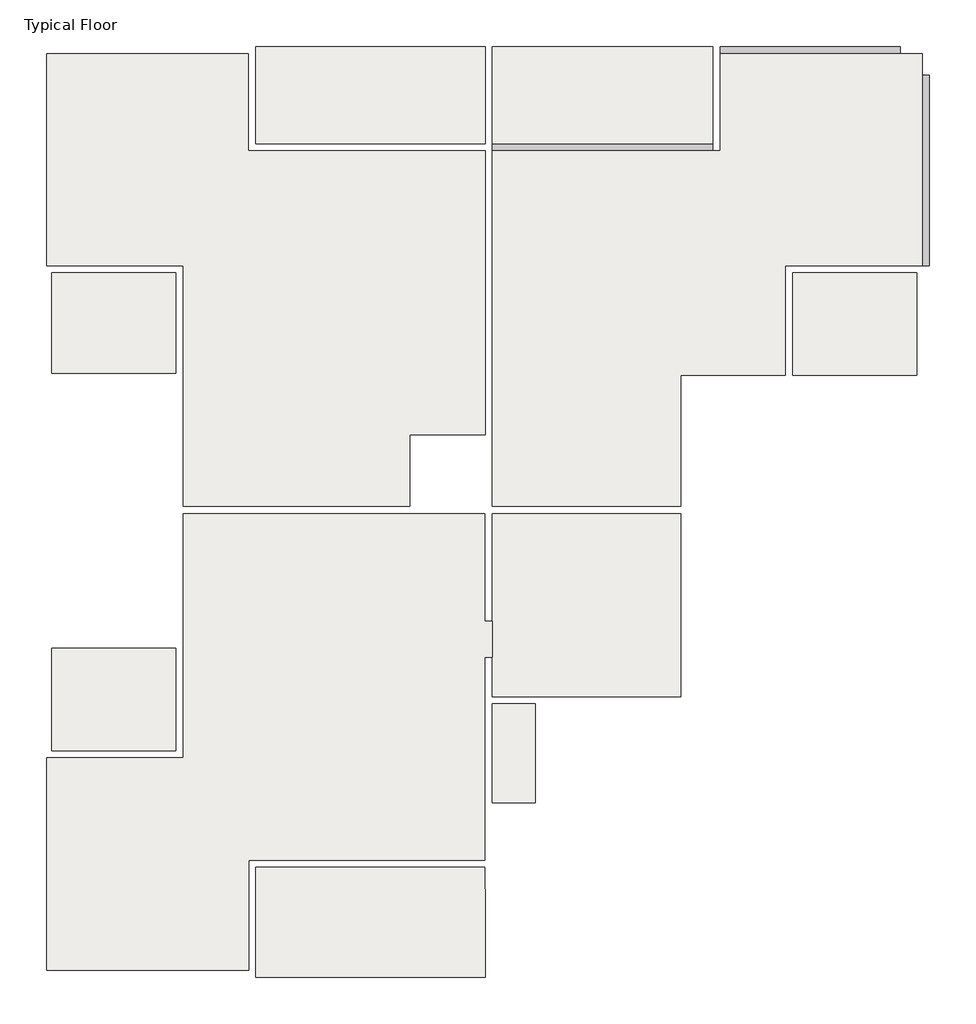
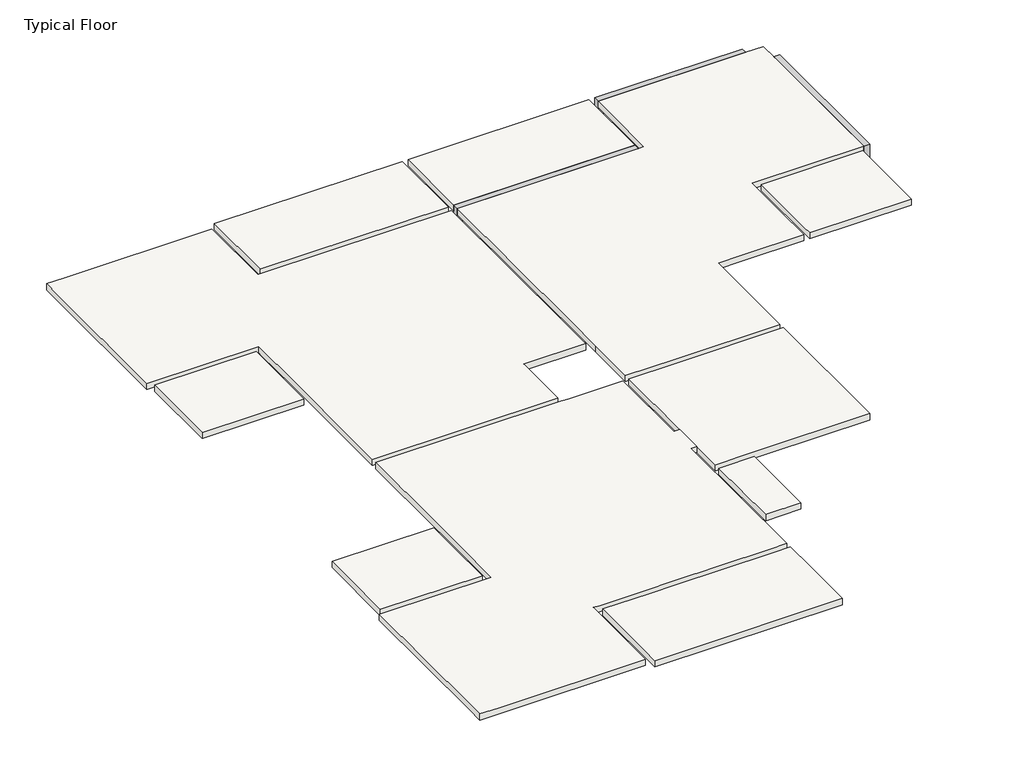
# One storey: 11 slabs, 3 beams.
"""IFC4 building model written with IfcOpenShell, lengths in millimetres."""

from ifc_helpers import new_model, si_unit, frame, origin, place, context, project, spatial, polyline, outline, extrude, faceted_brep, element, save

model = new_model("IFC4")

# Units and contexts
model_context = context("Model", 3, world=origin())
ifc_project = project(units=[si_unit("LENGTHUNIT", "METRE", prefix="MILLI")], contexts=[model_context])

# Site, building, storey
site = spatial("IfcSite", under=ifc_project)
building = spatial("IfcBuilding", under=site)
storey = spatial("IfcBuildingStorey", under=building, Name="Typical Floor", Elevation=3200.0)

# Beams
placement = place(None, origin())
element("IfcBeam", 1, ObjectType="Concrete Rectengular Beam : 20/50", at=placement, inside=storey, context=model_context, shape_type="Brep", body=[
    faceted_brep([(23241.1179501, 12375.8954895, 3200.0), (23241.1179501, 12575.8954895, 3200.0), (18221.404101, 12575.8954895, 3200.0), (18221.404101, 12375.8954895, 3200.0), (23241.1179501, 12375.8954895, 2700.0), (18221.404101, 12375.8954895, 2980.0), (18221.404101, 12375.8954895, 2700.0), (23241.1179501, 12575.8954895, 2700.0), (18221.404101, 12575.8954895, 2700.0)], [[[0, 1, 2, 3]], [[4, 0, 3, 5, 6]], [[7, 4, 6, 8]], [[1, 7, 8, 2]], [[1, 0, 4, 7]], [[3, 2, 8, 6, 5]]]),
])
element("IfcBeam", 2, ObjectType="Concrete Rectengular Beam : 20/50", at=placement, inside=storey, context=model_context, shape_type="Brep", body=[
    faceted_brep([(24041.1179501, 11775.8954895, 3200.0), (23841.1179501, 11775.8954895, 3200.0), (23841.1179501, 6476.2289939, 3200.0), (24041.1179501, 6476.2289939, 3200.0), (24041.1179501, 11775.8954895, 2700.0), (24041.1179501, 6476.2289939, 2700.0), (23841.1179501, 11775.8954895, 2700.0), (23841.1179501, 6476.2289939, 2700.0), (23841.1179501, 6476.2289939, 2980.0)], [[[0, 1, 2, 3]], [[4, 0, 3, 5]], [[6, 4, 5, 7]], [[1, 6, 7, 8, 2]], [[1, 0, 4, 6]], [[3, 2, 8, 7, 5]]]),
])
element("IfcBeam", 3, ObjectType="Concrete Rectengular Beam : 20/50", at=placement, inside=storey, context=model_context, shape_type="Brep", body=[
    faceted_brep([(11879.1824488, 9876.3316106, 3200.0), (11879.1824488, 9676.3316106, 3200.0), (18021.404101, 9676.3316106, 3200.0), (18021.404101, 9876.3316106, 3200.0), (11879.1824488, 9676.3316106, 2980.0), (11879.1824488, 9676.3316106, 2700.0), (18021.404101, 9676.3316106, 2700.0), (11879.1824488, 9876.3316106, 2700.0), (18021.404101, 9876.3316106, 2700.0), (11879.1824488, 9876.3316106, 2980.0), (18021.404101, 9876.3316106, 2980.0)], [[[0, 1, 2, 3]], [[1, 4, 5, 6, 2]], [[5, 7, 8, 6]], [[7, 9, 0, 3, 10, 8]], [[1, 0, 9, 7, 5, 4]], [[3, 2, 6, 8, 10]]]),
])

# Slabs
element("IfcSlab", 4, ObjectType="22", at=placement, inside=storey, context=model_context, shape_type="Brep", body=[
    faceted_brep([(11683.1306274, -13330.359, 2980.0), (11678.1306274, -13330.359, 2980.0), (5300.1419152, -13330.359, 2980.0), (5300.1419152, -10269.2815244, 2980.0), (11678.1306274, -10269.2815244, 2980.0), (11678.1306274, -10870.359, 2980.0), (11683.1306274, -10870.359, 2980.0), (5300.1419152, -13330.359, 3200.0), (11683.1306274, -13330.359, 3200.0), (11683.1306274, -10870.359, 3200.0), (11678.1306274, -10870.359, 3200.0), (11678.1306274, -10269.2815244, 3200.0), (11078.1049732, -10269.2815244, 3200.0), (7729.8494576, -10269.2815244, 3200.0), (6929.8238034, -10269.2815244, 3200.0), (5300.1419152, -10269.2815244, 3200.0)], [[[0, 1, 2, 3, 4, 5, 6]], [[7, 8, 9, 10, 11, 12, 13, 14, 15]], [[8, 0, 6, 9]], [[2, 1, 0, 8, 7]], [[3, 2, 7, 15]], [[3, 15, 14, 13, 12, 11, 4]], [[10, 5, 4, 11]], [[5, 10, 9, 6]]]),
])
element("IfcSlab", 5, ObjectType="22", at=placement, inside=storey, context=model_context, shape_type="Brep", body=[
    faceted_brep([(3076.7966099, -4169.8715705, 2980.0), (3076.7966099, -7021.5647465, 2980.0), (-373.331661, -7021.5647465, 2980.0), (-373.331661, -4169.8715705, 2980.0), (3076.7966099, -4169.8715705, 3200.0), (-373.331661, -4169.8715705, 3200.0), (-373.331661, -7021.5647465, 3200.0), (3076.7966099, -7021.5647465, 3200.0), (3076.7966099, -5270.1794207, 3200.0), (3076.7966099, -4470.1537665, 3200.0)], [[[0, 1, 2, 3]], [[4, 5, 6, 7, 8, 9]], [[1, 0, 4, 9, 8, 7]], [[2, 1, 7, 6]], [[3, 2, 6, 5]], [[0, 3, 5, 4]]]),
])
element("IfcSlab", 6, ObjectType="22", at=placement, inside=storey, context=model_context, shape_type="Brep", body=[
    faceted_brep([(23691.6965586, 3423.845178, 2980.0), (20241.5682877, 3423.845178, 2980.0), (20241.5682877, 6276.2289939, 2980.0), (23691.6965586, 6276.2289939, 2980.0), (23691.6965586, 3423.845178, 3200.0), (23691.6965586, 6276.2289939, 3200.0), (20241.5682877, 6276.2289939, 3200.0), (20241.5682877, 4529.076608, 3200.0), (20241.5682877, 3729.0509538, 3200.0), (20241.5682877, 3423.845178, 3200.0)], [[[0, 1, 2, 3]], [[4, 5, 6, 7, 8, 9]], [[1, 0, 4, 9]], [[2, 1, 9, 8, 7, 6]], [[3, 2, 6, 5]], [[0, 3, 5, 4]]]),
])
element("IfcSlab", 7, ObjectType="22", at=placement, inside=storey, context=model_context, shape_type="Brep", body=[
    faceted_brep([(3076.7966099, 6276.2289939, 2980.0), (3076.7966099, 3479.5640375, 2980.0), (-373.331661, 3479.5640375, 2980.0), (-373.331661, 6276.2289939, 2980.0), (3076.7966099, 6276.2289939, 3200.0), (-373.331661, 6276.2289939, 3200.0), (-373.331661, 3479.5640375, 3200.0), (3076.7966099, 3479.5640375, 3200.0), (3076.7966099, 3729.0509538, 3200.0), (3076.7966099, 4529.076608, 3200.0)], [[[0, 1, 2, 3]], [[4, 5, 6, 7, 8, 9]], [[1, 0, 4, 9, 8, 7]], [[2, 1, 7, 6]], [[3, 2, 6, 5]], [[0, 3, 5, 4]]]),
])
element("IfcSlab", 8, ObjectType="22", at=placement, inside=storey, context=model_context, shape_type="Brep", body=[
    faceted_brep([(11878.1306274, -5719.9228789, 2980.0), (13080.2855786, -5719.9228789, 2980.0), (13080.2855786, -8469.230216, 2980.0), (11878.1306274, -8469.230216, 2980.0), (13080.2855786, -5719.9228789, 3200.0), (11979.7211866, -5719.9228789, 3200.0), (11878.1306274, -5719.9228789, 3200.0), (11878.1306274, -8469.230216, 3200.0), (13080.2855786, -8469.230216, 3200.0)], [[[0, 1, 2, 3]], [[4, 5, 6, 7, 8]], [[1, 4, 8, 2]], [[6, 0, 3, 7]], [[1, 0, 6, 5, 4]], [[3, 2, 8, 7]]]),
])
element("IfcSlab", 9, ObjectType="22", at=placement, inside=storey, context=model_context, shape_type="Brep", body=[
    faceted_brep([(3276.7966099, -419.230216, 2980.0), (11678.1306274, -419.230216, 2980.0), (11678.1306274, -3420.3846542, 2980.0), (11878.1306274, -3420.3846542, 2980.0), (11878.1306274, -4419.3584869, 2980.0), (11678.1306274, -4419.3584869, 2980.0), (11678.1306274, -10069.2815244, 2980.0), (11078.1049732, -10069.2815244, 2980.0), (7729.8494576, -10069.2815244, 2980.0), (6929.8238034, -10069.2815244, 2980.0), (5300.1419152, -10069.2815244, 2980.0), (5100.1419152, -10069.2815244, 2980.0), (5100.1419152, -13130.7628896, 2980.0), (77.2469476, -13130.7628896, 2980.0), (-522.7530524, -13130.7628896, 2980.0), (-522.7530524, -12530.7628896, 2980.0), (-522.7530524, -7221.5647465, 2980.0), (-373.331661, -7221.5647465, 2980.0), (3276.7966099, -7221.5647465, 2980.0), (3276.7966099, -7021.5647465, 2980.0), (3276.7966099, -5270.1794207, 2980.0), (3276.7966099, -4470.1537665, 2980.0), (3276.7966099, -3919.8715705, 2980.0), (11678.1306274, -419.230216, 3200.0), (9829.6442241, -419.230216, 3200.0), (9579.6442241, -419.230216, 3200.0), (3276.7966099, -419.230216, 3200.0), (3276.7966099, -3919.8715705, 3200.0), (3276.7966099, -4470.1537665, 3200.0), (3276.7966099, -5270.1794207, 3200.0), (3276.7966099, -7021.5647465, 3200.0), (3276.7966099, -7221.5647465, 3200.0), (-373.331661, -7221.5647465, 3200.0), (-522.7530524, -7221.5647465, 3200.0), (-522.7530524, -12530.7628896, 3200.0), (-522.7530524, -13130.7628896, 3200.0), (77.2469476, -13130.7628896, 3200.0), (5100.1419152, -13130.7628896, 3200.0), (5100.1419152, -10069.2815244, 3200.0), (5300.1419152, -10069.2815244, 3200.0), (6929.8238034, -10069.2815244, 3200.0), (7729.8494576, -10069.2815244, 3200.0), (11078.1049732, -10069.2815244, 3200.0), (11678.1306274, -10069.2815244, 3200.0), (11678.1306274, -4419.3584869, 3200.0), (11878.1306274, -4419.3584869, 3200.0), (11878.1306274, -3420.3846542, 3200.0), (11678.1306274, -3420.3846542, 3200.0)], [[[0, 1, 2, 3, 4, 5, 6, 7, 8, 9, 10, 11, 12, 13, 14, 15, 16, 17, 18, 19, 20, 21, 22]], [[23, 24, 25, 26, 27, 28, 29, 30, 31, 32, 33, 34, 35, 36, 37, 38, 39, 40, 41, 42, 43, 44, 45, 46, 47]], [[31, 18, 17, 16, 33, 32]], [[18, 31, 30, 29, 28, 27, 26, 0, 22, 21, 20, 19]], [[1, 0, 26, 25, 24, 23]], [[2, 1, 23, 47]], [[3, 2, 47, 46]], [[4, 3, 46, 45]], [[5, 4, 45, 44]], [[6, 5, 44, 43]], [[6, 43, 42, 41, 40, 39, 38, 11, 10, 9, 8, 7]], [[12, 11, 38, 37]], [[12, 37, 36, 35, 14, 13]], [[14, 35, 34, 33, 16, 15]]]),
])
element("IfcSlab", 10, ObjectType="22", at=placement, inside=storey, context=model_context, shape_type="Brep", body=[
    faceted_brep([(17129.3735672, -420.2820374, 2980.0), (17129.3735672, -5519.9228789, 2980.0), (11878.1306274, -5519.9228789, 2980.0), (11878.1306274, -4419.3584869, 2980.0), (11878.1306274, -3420.3846542, 2980.0), (11878.1306274, -420.2820374, 2980.0), (17129.3735672, -420.2820374, 3200.0), (13528.9772154, -420.2820374, 3200.0), (11878.1306274, -420.2820374, 3200.0), (11878.1306274, -3420.3846542, 3200.0), (11878.1306274, -4419.3584869, 3200.0), (11878.1306274, -5519.9228789, 3200.0), (11979.7211866, -5519.9228789, 3200.0), (13080.2855786, -5519.9228789, 3200.0), (17129.3735672, -5519.9228789, 3200.0)], [[[0, 1, 2, 3, 4, 5]], [[6, 7, 8, 9, 10, 11, 12, 13, 14]], [[1, 0, 6, 14]], [[2, 1, 14, 13, 12, 11]], [[5, 4, 3, 2, 11, 10, 9, 8]], [[0, 5, 8, 7, 6]]]),
])
element("IfcSlab", 11, ObjectType="22", at=placement, inside=storey, context=model_context, shape_type="Brep", body=[
    faceted_brep([(11879.1824488, -220.2820374, 2980.0), (11879.1824488, 1527.9221698, 2980.0), (11879.1824488, 9676.3316106, 2980.0), (18021.404101, 9676.3316106, 2980.0), (18221.404101, 9676.3316106, 2980.0), (18221.404101, 12375.8954895, 2980.0), (23241.1179501, 12375.8954895, 2980.0), (23841.1179501, 12375.8954895, 2980.0), (23841.1179501, 11775.8954895, 2980.0), (23841.1179501, 6476.2289939, 2980.0), (20041.5682877, 6476.2289939, 2980.0), (20041.5682877, 6276.2289939, 2980.0), (20041.5682877, 4529.076608, 2980.0), (20041.5682877, 3729.0509538, 2980.0), (20041.5682877, 3423.845178, 2980.0), (17929.3735672, 3423.845178, 2980.0), (17129.3735672, 3423.845178, 2980.0), (17129.3735672, 2623.845178, 2980.0), (17129.3735672, -220.2820374, 2980.0), (11879.1824488, 1527.9221698, 3200.0), (11879.1824488, -220.2820374, 3200.0), (13528.9772154, -220.2820374, 3200.0), (17129.3735672, -220.2820374, 3200.0), (17129.3735672, 2623.845178, 3200.0), (17129.3735672, 3423.845178, 3200.0), (17929.3735672, 3423.845178, 3200.0), (20041.5682877, 3423.845178, 3200.0), (20041.5682877, 3729.0509538, 3200.0), (20041.5682877, 4529.076608, 3200.0), (20041.5682877, 6276.2289939, 3200.0), (20041.5682877, 6476.2289939, 3200.0), (23841.1179501, 6476.2289939, 3200.0), (23841.1179501, 11775.8954895, 3200.0), (23841.1179501, 12375.8954895, 3200.0), (23241.1179501, 12375.8954895, 3200.0), (18221.404101, 12375.8954895, 3200.0), (18221.404101, 9676.3316106, 3200.0), (18021.404101, 9676.3316106, 3200.0), (11879.1824488, 9676.3316106, 3200.0), (11879.1824488, 2979.8205793, 3200.0), (11879.1824488, 1976.6138066, 3200.0)], [[[0, 1, 2, 3, 4, 5, 6, 7, 8, 9, 10, 11, 12, 13, 14, 15, 16, 17, 18]], [[19, 20, 21, 22, 23, 24, 25, 26, 27, 28, 29, 30, 31, 32, 33, 34, 35, 36, 37, 38, 39, 40]], [[1, 0, 20, 19]], [[2, 1, 19, 40, 39, 38]], [[2, 38, 37, 36, 4, 3]], [[5, 4, 36, 35]], [[5, 35, 34, 33, 7, 6]], [[7, 33, 32, 31, 9, 8]], [[10, 9, 31, 30]], [[10, 30, 29, 28, 27, 26, 14, 13, 12, 11]], [[14, 26, 25, 24, 16, 15]], [[16, 24, 23, 22, 18, 17]], [[0, 18, 22, 21, 20]]]),
])
element("IfcSlab", 12, ObjectType="22", at=placement, inside=storey, context=model_context, shape_type="Brep", body=[
    faceted_brep([(5096.9607967, 12375.8954895, 2980.0), (5096.9607967, 9676.3316106, 2980.0), (5296.9607967, 9676.3316106, 2980.0), (11679.1824488, 9676.3316106, 2980.0), (11679.1824488, 1777.9221698, 2980.0), (9579.6442241, 1777.9221698, 2980.0), (9579.6442241, 1527.9221698, 2980.0), (9579.6442241, -219.230216, 2980.0), (3276.7966099, -219.230216, 2980.0), (3276.7966099, 3229.5640375, 2980.0), (3276.7966099, 3729.0509538, 2980.0), (3276.7966099, 4529.076608, 2980.0), (3276.7966099, 6276.2289939, 2980.0), (3276.7966099, 6476.2289939, 2980.0), (-522.7530524, 6476.2289939, 2980.0), (-522.7530524, 11775.8954895, 2980.0), (-522.7530524, 12375.8954895, 2980.0), (77.2469476, 12375.8954895, 2980.0), (5096.9607967, 9676.3316106, 3200.0), (5096.9607967, 12375.8954895, 3200.0), (77.2469476, 12375.8954895, 3200.0), (-522.7530524, 12375.8954895, 3200.0), (-522.7530524, 11775.8954895, 3200.0), (-522.7530524, 6476.2289939, 3200.0), (3276.7966099, 6476.2289939, 3200.0), (3276.7966099, 6276.2289939, 3200.0), (3276.7966099, 4529.076608, 3200.0), (3276.7966099, 3729.0509538, 3200.0), (3276.7966099, 3229.5640375, 3200.0), (3276.7966099, -219.230216, 3200.0), (9579.6442241, -219.230216, 3200.0), (9579.6442241, 1527.9221698, 3200.0), (9579.6442241, 1777.9221698, 3200.0), (11679.1824488, 1777.9221698, 3200.0), (11679.1824488, 1976.6138066, 3200.0), (11679.1824488, 2979.8205793, 3200.0), (11679.1824488, 9676.3316106, 3200.0), (5296.9607967, 9676.3316106, 3200.0)], [[[0, 1, 2, 3, 4, 5, 6, 7, 8, 9, 10, 11, 12, 13, 14, 15, 16, 17]], [[18, 19, 20, 21, 22, 23, 24, 25, 26, 27, 28, 29, 30, 31, 32, 33, 34, 35, 36, 37]], [[21, 16, 15, 14, 23, 22]], [[16, 21, 20, 19, 0, 17]], [[1, 0, 19, 18]], [[1, 18, 37, 36, 3, 2]], [[4, 3, 36, 35, 34, 33]], [[5, 4, 33, 32]], [[5, 32, 31, 30, 7, 6]], [[8, 7, 30, 29]], [[8, 29, 28, 27, 26, 25, 24, 13, 12, 11, 10, 9]], [[14, 13, 24, 23]]]),
])
element("IfcSlab", 13, ObjectType="22", at=placement, inside=storey, context=model_context, shape_type="SweptSolid", body=[
    extrude(outline(polyline([(18021.404101, 12575.8954895), (18021.404101, 9876.3316106), (11879.1824488, 9876.3316106), (11879.1824488, 12575.8954895), (18021.404101, 12575.8954895)])), frame((0.0, 0.0, 2980.0), z_axis=(0.0, 0.0, 1.0), x_axis=(1.0, 0.0, 0.0)), (0.0, 0.0, 1.0), 220.0),
])
element("IfcSlab", 14, ObjectType="22", at=placement, inside=storey, context=model_context, shape_type="SweptSolid", body=[
    extrude(outline(polyline([(5296.9607967, 12575.8954895), (11679.1824488, 12575.8954895), (11679.1824488, 9876.3316106), (5296.9607967, 9876.3316106), (5296.9607967, 12575.8954895)])), frame((0.0, 0.0, 2980.0), z_axis=(0.0, 0.0, 1.0), x_axis=(1.0, 0.0, 0.0)), (0.0, 0.0, 1.0), 220.0),
])

save(model, "model.ifc")

# Revit data of these elements
# Type "Concrete Rectengular Beam : 20/50"
#   Length [instance default] = 152.4 cm
#   b = 20 cm
#   h = 50 cm
#   Structural Material [instance default] = Concrete
#   Assembly Code = ""
# Type "22"
#   Function = 0
#   Layers, outside or top first: 22 cm "Concrete" (function 1)
# Element 1 (IfcBeam, "Concrete Rectengular Beam : 20/50")
#   Comments = ""
#   Mark = "B4"
#   SOFiSTiK_AMG_Comments = ""
#   SOFiSTiK_AMG_Scheduled = yes
#   SOFiSTiK_AMG_Adjusted = yes
#   Structural Material = Concrete
#   Phase Created = New Construction
#   Materials on its faces: "Concrete"
# Element 2 (IfcBeam, "Concrete Rectengular Beam : 20/50")
#   Comments = ""
#   Mark = "B5"
#   SOFiSTiK_AMG_Comments = ""
#   SOFiSTiK_AMG_Scheduled = yes
#   SOFiSTiK_AMG_Adjusted = yes
#   Structural Material = Concrete
#   Phase Created = New Construction
#   Materials on its faces: "Concrete"
# Element 3 (IfcBeam, "Concrete Rectengular Beam : 20/50")
#   Comments = ""
#   Mark = "B6"
#   SOFiSTiK_AMG_Comments = ""
#   SOFiSTiK_AMG_Scheduled = yes
#   SOFiSTiK_AMG_Adjusted = yes
#   Structural Material = Concrete
#   Phase Created = New Construction
#   Materials on its faces: "Concrete"
# Element 4 (IfcSlab, "22")
#   Mark = "S1"
#   SOFiSTiK_AMG_Comments = ""
#   Height Offset From Level = 0 cm
#   built-in parameter 1001954 = 1
#   SOFiSTiK_AMG_Scheduled = yes
#   SOFiSTiK_AMG_Adjusted = yes
#   Phase Created = New Construction
#   Materials on its faces: "Concrete"
# Element 5 (IfcSlab, "22")
#   Mark = "S2"
#   SOFiSTiK_AMG_Comments = ""
#   Height Offset From Level = 0 cm
#   built-in parameter 1001954 = 1
#   SOFiSTiK_AMG_Scheduled = yes
#   SOFiSTiK_AMG_Adjusted = yes
#   Phase Created = New Construction
#   Materials on its faces: "Concrete"
# Element 6 (IfcSlab, "22")
#   Mark = "S3"
#   SOFiSTiK_AMG_Comments = ""
#   Height Offset From Level = 0 cm
#   built-in parameter 1001954 = 1
#   SOFiSTiK_AMG_Scheduled = yes
#   SOFiSTiK_AMG_Adjusted = yes
#   Phase Created = New Construction
#   Materials on its faces: "Concrete"
# Element 7 (IfcSlab, "22")
#   Mark = "S4"
#   SOFiSTiK_AMG_Comments = ""
#   Height Offset From Level = 0 cm
#   built-in parameter 1001954 = 1
#   SOFiSTiK_AMG_Scheduled = yes
#   SOFiSTiK_AMG_Adjusted = yes
#   Phase Created = New Construction
#   Materials on its faces: "Concrete"
# Element 8 (IfcSlab, "22")
#   Mark = "S5"
#   SOFiSTiK_AMG_Comments = ""
#   Height Offset From Level = 0 cm
#   built-in parameter 1001954 = 1
#   SOFiSTiK_AMG_Scheduled = yes
#   SOFiSTiK_AMG_Adjusted = yes
#   Phase Created = New Construction
#   Materials on its faces: "Concrete"
# Element 9 (IfcSlab, "22")
#   Mark = "S6"
#   SOFiSTiK_AMG_Comments = ""
#   built-in parameter 1001955 = 1.5708 (stored number, unit not read)
#   Height Offset From Level = 0 cm
#   built-in parameter 1001954 = 1
#   SOFiSTiK_AMG_Scheduled = yes
#   SOFiSTiK_AMG_Adjusted = yes
#   Phase Created = New Construction
#   Materials on its faces: "Concrete"
# Element 10 (IfcSlab, "22")
#   Mark = "S7"
#   SOFiSTiK_AMG_Comments = ""
#   Height Offset From Level = 0 cm
#   built-in parameter 1001954 = 1
#   SOFiSTiK_AMG_Scheduled = yes
#   SOFiSTiK_AMG_Adjusted = yes
#   Phase Created = New Construction
#   Materials on its faces: "Concrete"
# Element 11 (IfcSlab, "22")
#   Mark = "S8"
#   SOFiSTiK_AMG_Comments = ""
#   built-in parameter 1001955 = -1.5708 (stored number, unit not read)
#   Height Offset From Level = 0 cm
#   built-in parameter 1001954 = 1
#   SOFiSTiK_AMG_Scheduled = yes
#   SOFiSTiK_AMG_Adjusted = yes
#   Phase Created = New Construction
#   Materials on its faces: "Concrete"
# Element 12 (IfcSlab, "22")
#   Mark = "S9"
#   SOFiSTiK_AMG_Comments = ""
#   built-in parameter 1001955 = -1.5708 (stored number, unit not read)
#   Height Offset From Level = 0 cm
#   built-in parameter 1001954 = 1
#   SOFiSTiK_AMG_Scheduled = yes
#   SOFiSTiK_AMG_Adjusted = yes
#   Phase Created = New Construction
#   Materials on its faces: "Concrete"
# Element 13 (IfcSlab, "22")
#   Mark = "S10"
#   SOFiSTiK_AMG_Comments = ""
#   Height Offset From Level = 0 cm
#   built-in parameter 1001954 = 1
#   SOFiSTiK_AMG_Scheduled = yes
#   SOFiSTiK_AMG_Adjusted = yes
#   Phase Created = New Construction
#   Materials on its faces: "Concrete"
# Element 14 (IfcSlab, "22")
#   Mark = "S11"
#   SOFiSTiK_AMG_Comments = ""
#   built-in parameter 1001955 = 3.14159 (stored number, unit not read)
#   Height Offset From Level = 0 cm
#   built-in parameter 1001954 = 1
#   SOFiSTiK_AMG_Scheduled = yes
#   SOFiSTiK_AMG_Adjusted = yes
#   Phase Created = New Construction
#   Materials on its faces: "Concrete"
# Materials
#   "Concrete": class "Concrete", colour RGB 192 192 192, transparency 0, Keynote = "01000", Description = "Cast-in-place concrete", Cost = 0
